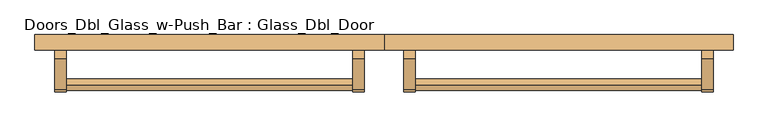
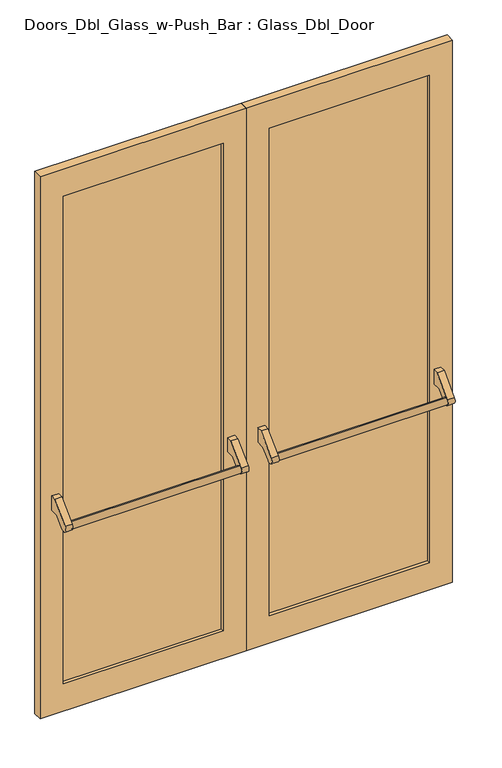
"""IFC4 building model written with IfcOpenShell, lengths in millimetres: door geometry, Doors_Dbl_Glass_w-Push_Bar : Glass_Dbl_Door."""

from ifc_helpers import new_model, si_unit, point, frame, frame_2d, origin, place, context, project, spatial, polyline, circle_curve, trimmed, segment, composite_curve, outline, extrude, source, transform, mapped, element, save


def doors_dbl_glass_w_push_bar_glass_dbl_door_d6e68b66(model_context):
    return source(origin(), model_context, "Body", "SweptSolid", [
        extrude(outline(composite_curve([segment(trimmed(circle_curve(frame_2d((-65.0203019, 909.5721086)), 15.0), [point((-65.0203019, 924.5721086))], [point((-65.0203019, 894.5721086))], False, "CARTESIAN"), True, "CONTINUOUS"), segment(trimmed(circle_curve(frame_2d((-65.0203019, 909.5721086)), 15.0), [point((-65.0203019, 894.5721086))], [point((-65.0203019, 924.5721086))], False, "CARTESIAN"), True, "CONTINUOUS")], self_intersect=False)), frame((80.0, 0.0, 0.0), z_axis=(1.0, 0.0, 0.0), x_axis=(0.0, 1.0, 0.0)), (0.0, 0.0, 1.0), 730.0),
        extrude(outline(composite_curve([segment(polyline([(0.1563269, 1000.0), (24.035259, 1000.0), (24.035259, 935.0), (-14.3411478, 935.0), (-52.3946705, 896.9464773)]), True, "CONTINUOUS"), segment(trimmed(circle_curve(frame_2d((-65.0203019, 909.5721086)), 17.8553391), [point((-52.3946705, 896.9464773))], [point((-77.6459332, 922.19774))], False, "CARTESIAN"), True, "CONTINUOUS"), segment(polyline([(-77.6459332, 922.19774), (0.1563269, 1000.0)]), True, "CONTINUOUS")], self_intersect=False)), frame((810.0, 0.0, 0.0), z_axis=(1.0, 0.0, 0.0), x_axis=(0.0, 1.0, 0.0)), (0.0, 0.0, 1.0), 30.0),
        extrude(outline(composite_curve([segment(polyline([(0.1563269, 1000.0), (24.035259, 1000.0), (24.035259, 935.0), (-14.3411478, 935.0), (-52.3946705, 896.9464773)]), True, "CONTINUOUS"), segment(trimmed(circle_curve(frame_2d((-65.0203019, 909.5721086)), 17.8553391), [point((-52.3946705, 896.9464773))], [point((-77.6459332, 922.19774))], False, "CARTESIAN"), True, "CONTINUOUS"), segment(polyline([(-77.6459332, 922.19774), (0.1563269, 1000.0)]), True, "CONTINUOUS")], self_intersect=False)), frame((50.0, 0.0, 0.0), z_axis=(1.0, 0.0, 0.0), x_axis=(0.0, 1.0, 0.0)), (0.0, 0.0, 1.0), 30.0),
        extrude(outline(composite_curve([segment(trimmed(circle_curve(frame_2d((-65.0203019, 909.5721086)), 15.0), [point((-65.0203019, 924.5721086))], [point((-65.0203019, 894.5721086))], False, "CARTESIAN"), True, "CONTINUOUS"), segment(trimmed(circle_curve(frame_2d((-65.0203019, 909.5721086)), 15.0), [point((-65.0203019, 894.5721086))], [point((-65.0203019, 924.5721086))], False, "CARTESIAN"), True, "CONTINUOUS")], self_intersect=False)), frame((-810.0, 0.0, 0.0), z_axis=(1.0, 0.0, 0.0), x_axis=(0.0, 1.0, 0.0)), (0.0, 0.0, 1.0), 730.0),
        extrude(outline(composite_curve([segment(polyline([(0.1563269, 1000.0), (24.035259, 1000.0), (24.035259, 935.0), (-14.3411478, 935.0), (-52.3946705, 896.9464773)]), True, "CONTINUOUS"), segment(trimmed(circle_curve(frame_2d((-65.0203019, 909.5721086)), 17.8553391), [point((-52.3946705, 896.9464773))], [point((-77.6459332, 922.19774))], False, "CARTESIAN"), True, "CONTINUOUS"), segment(polyline([(-77.6459332, 922.19774), (0.1563269, 1000.0)]), True, "CONTINUOUS")], self_intersect=False)), frame((-80.0, 0.0, 0.0), z_axis=(1.0, 0.0, 0.0), x_axis=(0.0, 1.0, 0.0)), (0.0, 0.0, 1.0), 30.0),
        extrude(outline(composite_curve([segment(polyline([(0.1563269, 1000.0), (24.035259, 1000.0), (24.035259, 935.0), (-14.3411478, 935.0), (-52.3946705, 896.9464773)]), True, "CONTINUOUS"), segment(trimmed(circle_curve(frame_2d((-65.0203019, 909.5721086)), 17.8553391), [point((-52.3946705, 896.9464773))], [point((-77.6459332, 922.19774))], False, "CARTESIAN"), True, "CONTINUOUS"), segment(polyline([(-77.6459332, 922.19774), (0.1563269, 1000.0)]), True, "CONTINUOUS")], self_intersect=False)), frame((-840.0, 0.0, 0.0), z_axis=(1.0, 0.0, 0.0), x_axis=(0.0, 1.0, 0.0)), (0.0, 0.0, 1.0), 30.0),
        extrude(outline(polyline([(2475.0, -890.0), (0.0, -890.0), (0.0, 0.0), (2475.0, 0.0), (2475.0, -890.0)]), holes=[polyline([(2350.0, -790.0), (2350.0, -100.0), (125.0, -100.0), (125.0, -790.0), (2350.0, -790.0)])]), frame((0.0, 24.035259, 0.0), z_axis=(0.0, 1.0, 0.0), x_axis=(0.0, 0.0, 1.0)), (0.0, 0.0, 1.0), 38.5435966),
        extrude(outline(polyline([(2475.0, 0.0), (0.0, 0.0), (0.0, 890.0), (2475.0, 890.0), (2475.0, 0.0)]), holes=[polyline([(2350.0, 100.0), (2350.0, 790.0), (125.0, 790.0), (125.0, 100.0), (2350.0, 100.0)])]), frame((0.0, 24.035259, 0.0), z_axis=(0.0, 1.0, 0.0), x_axis=(0.0, 0.0, 1.0)), (0.0, 0.0, 1.0), 38.5435966),
        extrude(outline(polyline([(-100.0, 38.0), (-790.0, 38.0), (-790.0, 50.0), (-100.0, 50.0), (-100.0, 38.0)])), frame((0.0, 0.0, 125.0), z_axis=(0.0, 0.0, 1.0), x_axis=(1.0, 0.0, 0.0)), (0.0, 0.0, 1.0), 2225.0),
        extrude(outline(polyline([(790.0, 38.0), (100.0, 38.0), (100.0, 50.0), (790.0, 50.0), (790.0, 38.0)])), frame((0.0, 0.0, 125.0), z_axis=(0.0, 0.0, 1.0), x_axis=(1.0, 0.0, 0.0)), (0.0, 0.0, 1.0), 2225.0),
    ])


if __name__ == "__main__":
    model = new_model("IFC4")
    model_context = context("Model", 3, world=origin())
    ifc_project = project(units=[si_unit("LENGTHUNIT", "METRE", prefix="MILLI")], contexts=[model_context])
    site = spatial("IfcSite", under=ifc_project)
    building = spatial("IfcBuilding", under=site)
    placement = place(None, origin())
    doors_dbl_glass_w_push_bar_glass_dbl_door_shape = doors_dbl_glass_w_push_bar_glass_dbl_door_d6e68b66(model_context)
    element("IfcDoor", 1, ObjectType="Doors_Dbl_Glass_w-Push_Bar : Glass_Dbl_Door", at=placement, inside=building, context=model_context, shape_type="MappedRepresentation", body=[
        mapped(doors_dbl_glass_w_push_bar_glass_dbl_door_shape, transform((0.0, 0.0, 0.0), x_axis=(1.0, 0.0, 0.0), y_axis=(0.0, 1.0, 0.0), z_axis=(0.0, 0.0, 1.0))),
    ])
    save(model, "model.ifc")

# Revit data of these elements
# Type "Doors_Dbl_Glass_w-Push_Bar : Glass_Dbl_Door"
#   Type Mark = "46"
#   Construction Type Id = "GSP4R"
#   Analytic Construction = "1/8 in Pilkington single glazing"
#   Visual Light Transmittance = 0.9
#   TopRail = 125 mm
#   Solar Heat Gain Coefficient = 0.78
#   Offset = 50 mm
#   MuntinRail = 100 mm
#   LockRail = 100 mm
#   Heat Transfer Coefficient (U) = 3.6886 W/(m²·K)
#   Handle Z Distance = 1000 mm
#   Handle X Offset = 65 mm
#   Glass Thickness = 12 mm
#   BottomRail = 125 mm
#   Material Ironmongery = Metal - Aluminum
#   Material Door = Metal - Aluminum
#   Material Glass = Glass
#   Function = (empty or 0)
# Element 1 (IfcDoor, "Doors_Dbl_Glass_w-Push_Bar : Glass_Dbl_Door")
#   Materials on its faces: "Metal - Aluminum", "Glass"
# Materials
#   "Metal - Aluminum": class "Metal", colour RGB 247 247 247, transparency 0
#   "Glass": class "Glass", colour RGB 0 128 192, transparency 0.9, Description = "Soda Lime Glass", Cost = 0
